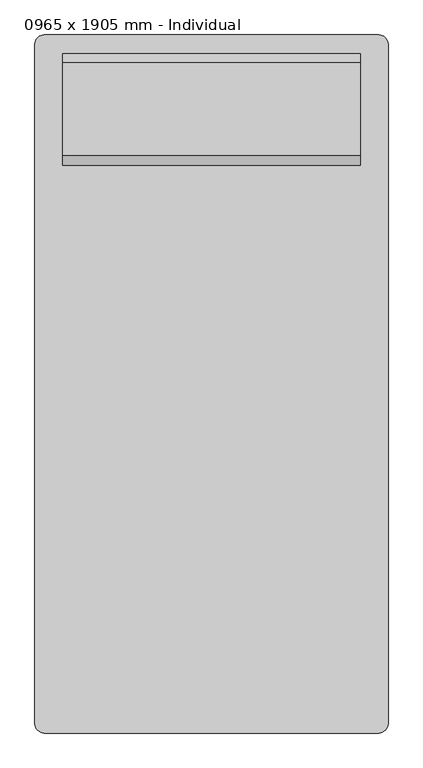
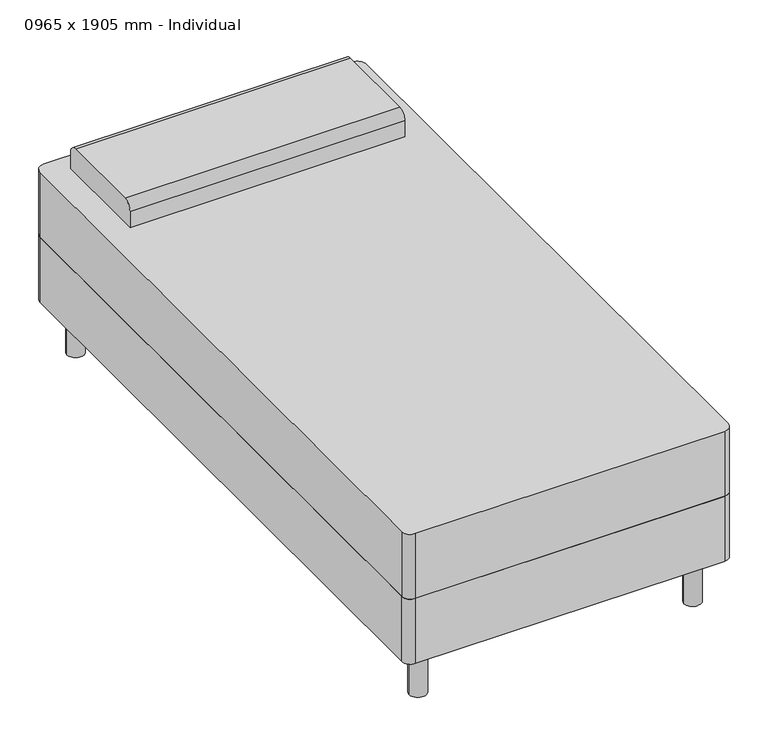
"""IFC4 building model written with IfcOpenShell, lengths in millimetres: furniture geometry, Cama-Estándar : 0965 x 1905 mm - Individual."""

import ifcopenshell
import ifcopenshell.guid

model = None  # the IFC model being written
_history = None  # IfcOwnerHistory: only IFC2X3 demands one
_inside = {}  # id of a spatial element -> (the spatial element, [elements in it])
_under = {}  # id of a project, library or spatial element -> (it, [spatial elements below it])
_declared = {}  # id of a project -> (the project, [libraries it declares])
_typed = {}  # id of a type object -> (the type object, [elements of that type])
_made_of = {}  # id of a material, layer set ... -> (it, [elements and type objects made of it])


def new_model(schema):
    """Start an empty IFC model of exactly this schema.

    Asked for "IFC4X3", IfcOpenShell would pick the latest addendum, in which some entities
    have other attributes; the version numbers below select the first issue.
    IFC2X3 requires an IfcOwnerHistory on every rooted entity: one is made here for all.
    """
    global model, _history
    if schema == "IFC4X3":
        model = ifcopenshell.file(schema_version=(4, 3, 0, 0))
    else:
        model = ifcopenshell.file(schema=schema)
    _inside.clear()
    _under.clear()
    _declared.clear()
    _typed.clear()
    _made_of.clear()
    _history = None
    if model.schema == "IFC2X3":
        org = make("IfcOrganization", Name="unknown")
        user = make(
            "IfcPersonAndOrganization",
            ThePerson=make("IfcPerson", FamilyName="unknown"),
            TheOrganization=org,
        )
        app = make(
            "IfcApplication",
            ApplicationDeveloper=org,
            Version="unknown",
            ApplicationFullName="unknown",
            ApplicationIdentifier="unknown",
        )
        _history = make(
            "IfcOwnerHistory",
            OwningUser=user,
            OwningApplication=app,
            ChangeAction="ADDED",
            CreationDate=0,
        )
    return model


def make(cls, **values):
    """One entity of the class cls with the attributes given. An attribute that is None is left unset."""
    return model.create_entity(
        cls, **{name: value for name, value in values.items() if value is not None}
    )


def rooted(cls, **values):
    """An entity with a GlobalId (a new one), such as an element, a storey or a relation."""
    return make(cls, GlobalId=ifcopenshell.guid.new(), OwnerHistory=_history, **values)


def si_unit(unit_type, name, prefix=None):
    """IfcSIUnit, for example si_unit("LENGTHUNIT", "METRE", prefix="MILLI")."""
    return make("IfcSIUnit", UnitType=unit_type, Prefix=prefix, Name=name)


def assignment(units):
    """IfcUnitAssignment: the units of a project."""
    return None if units is None else make("IfcUnitAssignment", Units=units)


def point(xyz):
    """IfcCartesianPoint."""
    return None if xyz is None else make("IfcCartesianPoint", Coordinates=xyz)


def direction(xyz):
    """IfcDirection."""
    return None if xyz is None else make("IfcDirection", DirectionRatios=xyz)


def frame(location, z_axis=None, x_axis=None):
    """IfcAxis2Placement3D, a coordinate frame: its origin and axes. An axis left out is left unset."""
    return make(
        "IfcAxis2Placement3D",
        Location=point(location),
        Axis=direction(z_axis),
        RefDirection=direction(x_axis),
    )


def frame_2d(location, x_axis=None):
    """IfcAxis2Placement2D, a coordinate frame in the plane: its origin and x axis."""
    return make(
        "IfcAxis2Placement2D", Location=point(location), RefDirection=direction(x_axis)
    )


def origin():
    """The frame at (0, 0, 0) with its axes left unset."""
    return frame((0.0, 0.0, 0.0))


def origin_with_axes():
    """The frame at (0, 0, 0) with the z axis (0, 0, 1) and the x axis (1, 0, 0) written out."""
    return frame((0.0, 0.0, 0.0), z_axis=(0.0, 0.0, 1.0), x_axis=(1.0, 0.0, 0.0))


def place(relative_to, where):
    """IfcLocalPlacement: puts the frame where relative to a parent placement (None: the world)."""
    return make(
        "IfcLocalPlacement", PlacementRelTo=relative_to, RelativePlacement=where
    )


def context(
    kind, dimensions, precision=None, world=None, true_north=None, identifier=None
):
    """IfcGeometricRepresentationContext, for example the 3D "Model" context."""
    return make(
        "IfcGeometricRepresentationContext",
        ContextIdentifier=identifier,
        ContextType=kind,
        CoordinateSpaceDimension=dimensions,
        Precision=precision,
        WorldCoordinateSystem=world,
        TrueNorth=true_north,
    )


def project(units=None, contexts=None):
    """IfcProject with its units and contexts."""
    return rooted(
        "IfcProject",
        Name="project",
        RepresentationContexts=contexts,
        UnitsInContext=assignment(units),
    )


def spatial(cls, under=None, at=None, **own):
    """A site, building, storey or space (cls), placed at a placement, below another one or the project."""
    s = rooted(cls, ObjectPlacement=at, **own)
    if under is not None:
        _under.setdefault(under.id(), (under, []))[1].append(s)
    return s


def polyline(points):
    """IfcPolyline through the points."""
    return make("IfcPolyline", Points=[point(p) for p in points])


def circle_curve(where, radius):
    """IfcCircle in the frame where."""
    return make("IfcCircle", Position=where, Radius=radius)


def trimmed(basis, trim1, trim2, sense, master):
    """IfcTrimmedCurve: the piece of a basis curve between two trims."""
    return make(
        "IfcTrimmedCurve",
        BasisCurve=basis,
        Trim1=trim1,
        Trim2=trim2,
        SenseAgreement=sense,
        MasterRepresentation=master,
    )


def segment(curve, same_sense, transition):
    """IfcCompositeCurveSegment."""
    return make(
        "IfcCompositeCurveSegment",
        Transition=transition,
        SameSense=same_sense,
        ParentCurve=curve,
    )


def composite_curve(segments, self_intersect=None):
    """IfcCompositeCurve: segments joined end to end."""
    return make("IfcCompositeCurve", Segments=segments, SelfIntersect=self_intersect)


def outline(outer, holes=None, kind="AREA"):
    """IfcArbitraryClosedProfileDef: a profile drawn as a closed curve; with holes, ...WithVoids."""
    if holes is None:
        return make("IfcArbitraryClosedProfileDef", ProfileType=kind, OuterCurve=outer)
    return make(
        "IfcArbitraryProfileDefWithVoids",
        ProfileType=kind,
        OuterCurve=outer,
        InnerCurves=holes,
    )


def extrude(swept, where, along, depth):
    """IfcExtrudedAreaSolid: the profile swept, set in the frame where, extruded along a direction by depth."""
    return make(
        "IfcExtrudedAreaSolid",
        SweptArea=swept,
        Position=where,
        ExtrudedDirection=direction(along),
        Depth=depth,
    )


def shape(context_of_items, identifier, shape_type, items):
    """IfcShapeRepresentation: the items that make up one representation, for example the "Body"."""
    return make(
        "IfcShapeRepresentation",
        ContextOfItems=context_of_items,
        RepresentationIdentifier=identifier,
        RepresentationType=shape_type,
        Items=items,
    )


def source(mapping_origin, context_of_items, identifier, shape_type, items):
    """IfcRepresentationMap: a shape defined once, which mapped items show again and again."""
    return make(
        "IfcRepresentationMap",
        MappingOrigin=mapping_origin,
        MappedRepresentation=shape(context_of_items, identifier, shape_type, items),
    )


def transform(
    local_origin,
    x_axis=None,
    y_axis=None,
    z_axis=None,
    scale=None,
    scale2=None,
    scale3=None,
    uniform=True,
):
    """IfcCartesianTransformationOperator3D, or its non-uniform kind. x_axis, y_axis, z_axis: its Axis1, 2, 3."""
    if uniform:
        return make(
            "IfcCartesianTransformationOperator3D",
            Axis1=direction(x_axis),
            Axis2=direction(y_axis),
            LocalOrigin=point(local_origin),
            Scale=scale,
            Axis3=direction(z_axis),
        )
    return make(
        "IfcCartesianTransformationOperator3DnonUniform",
        Axis1=direction(x_axis),
        Axis2=direction(y_axis),
        LocalOrigin=point(local_origin),
        Scale=scale,
        Axis3=direction(z_axis),
        Scale2=scale2,
        Scale3=scale3,
    )


def mapped(mapping_source, mapping_target):
    """IfcMappedItem: shows the shape of a source again, moved by a transform."""
    return make(
        "IfcMappedItem", MappingSource=mapping_source, MappingTarget=mapping_target
    )


def made_of(thing, what):
    """Note that an element or type object is made of a material, layer set ...; save() writes the relation."""
    if what is not None:
        _made_of.setdefault(what.id(), (what, []))[1].append(thing)
    return thing


def element(
    cls,
    number,
    at=None,
    inside=None,
    cuts=None,
    type_object=None,
    material=None,
    context=None,
    identifier="Body",
    shape_type=None,
    held_by="IfcProductDefinitionShape",
    body=None,
    shapes=None,
    **own,
):
    """One element of the class cls, such as IfcWall. Its Tag is "e" and its number.

    at: its placement. inside: the storey or other place that contains it. cuts: it is an
    opening in that element (IfcRelVoidsElement). A single representation is given by context,
    identifier, shape_type and body (its items); several are given by shapes. held_by: the class
    of the entity that holds the representations. save() writes the other relations.
    """
    e = rooted(cls, Tag="e%d" % number, ObjectPlacement=at, **own)
    if body is not None:
        shapes = [shape(context, identifier, shape_type, body)]
    if shapes is not None:
        e.Representation = make(held_by, Representations=shapes)
    if inside is not None:
        _inside.setdefault(inside.id(), (inside, []))[1].append(e)
    if cuts is not None:
        rooted(
            "IfcRelVoidsElement", RelatingBuildingElement=cuts, RelatedOpeningElement=e
        )
    if type_object is not None:
        _typed.setdefault(type_object.id(), (type_object, []))[1].append(e)
    return made_of(e, material)


def aggregate(whole, parts):
    """IfcRelAggregates: a whole, such as a stair, and the parts it consists of."""
    return rooted("IfcRelAggregates", RelatingObject=whole, RelatedObjects=parts)


def save(model, path):
    """Write the relations noted so far, then the file.

    IfcRelAggregates (storeys below a building ...), IfcRelContainedInSpatialStructure (elements
    in a storey), IfcRelDefinesByType, IfcRelAssociatesMaterial and IfcRelDeclares: one each for
    every whole, place, type object, material and project.
    """
    for whole, parts in _under.values():
        aggregate(whole, parts)
    for where, things in _inside.values():
        rooted(
            "IfcRelContainedInSpatialStructure",
            RelatedElements=things,
            RelatingStructure=where,
        )
    for kind, things in _typed.values():
        rooted("IfcRelDefinesByType", RelatedObjects=things, RelatingType=kind)
    for what, things in _made_of.values():
        rooted("IfcRelAssociatesMaterial", RelatedObjects=things, RelatingMaterial=what)
    for by, libraries in _declared.values():
        rooted("IfcRelDeclares", RelatingContext=by, RelatedDefinitions=libraries)
    model.write(path)


def furniture_0965_x_1905_mm_individual_fc46863d(model_context):
    return source(origin(), model_context, "Body", "SweptSolid", [
        extrude(outline(composite_curve([segment(polyline([(-211.0114754, -972.695082), (-211.0114754, 881.504918)]), True, "CONTINUOUS"), segment(trimmed(circle_curve(frame_2d((-185.6114754, 881.504918)), 25.4), [point((-211.0114754, 881.504918))], [point((-185.6114754, 906.904918))], False, "CARTESIAN"), True, "CONTINUOUS"), segment(polyline([(-185.6114754, 906.904918), (728.5885246, 906.904918)]), True, "CONTINUOUS"), segment(trimmed(circle_curve(frame_2d((728.5885246, 881.504918)), 25.4), [point((728.5885246, 906.904918))], [point((753.9885246, 881.504918))], False, "CARTESIAN"), True, "CONTINUOUS"), segment(polyline([(753.9885246, 881.504918), (753.9885246, -972.695082)]), True, "CONTINUOUS"), segment(trimmed(circle_curve(frame_2d((728.5885246, -972.695082)), 25.4), [point((753.9885246, -972.695082))], [point((728.5885246, -998.095082))], False, "CARTESIAN"), True, "CONTINUOUS"), segment(polyline([(728.5885246, -998.095082), (-185.6114754, -998.095082)]), True, "CONTINUOUS"), segment(trimmed(circle_curve(frame_2d((-185.6114754, -972.695082)), 25.4), [point((-185.6114754, -998.095082))], [point((-211.0114754, -972.695082))], False, "CARTESIAN"), True, "CONTINUOUS")], self_intersect=False)), frame((0.0, 0.0, 152.4), z_axis=(0.0, 0.0, 1.0), x_axis=(1.0, 0.0, 0.0)), (0.0, 0.0, 1.0), 203.2),
        extrude(outline(composite_curve([segment(polyline([(551.304918, 558.8), (551.304918, 609.6)]), True, "CONTINUOUS"), segment(trimmed(circle_curve(frame_2d((576.704918, 609.6)), 25.4), [point((551.304918, 609.6))], [point((576.704918, 635.0))], False, "CARTESIAN"), True, "CONTINUOUS"), segment(polyline([(576.704918, 635.0), (830.704918, 635.0)]), True, "CONTINUOUS"), segment(trimmed(circle_curve(frame_2d((830.704918, 609.6)), 25.4), [point((830.704918, 635.0))], [point((856.104918, 609.6))], False, "CARTESIAN"), True, "CONTINUOUS"), segment(polyline([(856.104918, 609.6), (856.104918, 558.8), (551.304918, 558.8)]), True, "CONTINUOUS")], self_intersect=False)), frame((-134.8114754, 0.0, 0.0), z_axis=(1.0, 0.0, 0.0), x_axis=(0.0, 1.0, 0.0)), (0.0, 0.0, 1.0), 812.6),
        extrude(outline(composite_curve([segment(trimmed(circle_curve(frame_2d((-134.8114754, 830.704918)), 25.4), [point((-160.2114754, 830.704918))], [point((-109.4114754, 830.704918))], False, "CARTESIAN"), True, "CONTINUOUS"), segment(trimmed(circle_curve(frame_2d((-134.8114754, 830.704918)), 25.4), [point((-109.4114754, 830.704918))], [point((-160.2114754, 830.704918))], False, "CARTESIAN"), True, "CONTINUOUS")], self_intersect=False)), origin_with_axes(), (0.0, 0.0, 1.0), 152.4),
        extrude(outline(composite_curve([segment(trimmed(circle_curve(frame_2d((677.7885246, 830.704918)), 25.4), [point((652.3885246, 830.704918))], [point((703.1885246, 830.704918))], False, "CARTESIAN"), True, "CONTINUOUS"), segment(trimmed(circle_curve(frame_2d((677.7885246, 830.704918)), 25.4), [point((703.1885246, 830.704918))], [point((652.3885246, 830.704918))], False, "CARTESIAN"), True, "CONTINUOUS")], self_intersect=False)), origin_with_axes(), (0.0, 0.0, 1.0), 152.4),
        extrude(outline(composite_curve([segment(trimmed(circle_curve(frame_2d((677.7885246, -921.895082)), 25.4), [point((652.3885246, -921.895082))], [point((703.1885246, -921.895082))], False, "CARTESIAN"), True, "CONTINUOUS"), segment(trimmed(circle_curve(frame_2d((677.7885246, -921.895082)), 25.4), [point((703.1885246, -921.895082))], [point((652.3885246, -921.895082))], False, "CARTESIAN"), True, "CONTINUOUS")], self_intersect=False)), origin_with_axes(), (0.0, 0.0, 1.0), 152.4),
        extrude(outline(composite_curve([segment(trimmed(circle_curve(frame_2d((-134.8114754, -921.895082)), 25.4), [point((-160.2114754, -921.895082))], [point((-109.4114754, -921.895082))], False, "CARTESIAN"), True, "CONTINUOUS"), segment(trimmed(circle_curve(frame_2d((-134.8114754, -921.895082)), 25.4), [point((-109.4114754, -921.895082))], [point((-160.2114754, -921.895082))], False, "CARTESIAN"), True, "CONTINUOUS")], self_intersect=False)), origin_with_axes(), (0.0, 0.0, 1.0), 152.4),
        extrude(outline(composite_curve([segment(polyline([(-185.6114754, 906.904918), (728.5885246, 906.904918)]), True, "CONTINUOUS"), segment(trimmed(circle_curve(frame_2d((728.5885246, 881.504918)), 25.4), [point((728.5885246, 906.904918))], [point((753.9885246, 881.504918))], False, "CARTESIAN"), True, "CONTINUOUS"), segment(polyline([(753.9885246, 881.504918), (753.9885246, -972.695082)]), True, "CONTINUOUS"), segment(trimmed(circle_curve(frame_2d((728.5885246, -972.695082)), 25.4), [point((753.9885246, -972.695082))], [point((728.5885246, -998.095082))], False, "CARTESIAN"), True, "CONTINUOUS"), segment(polyline([(728.5885246, -998.095082), (-185.6114754, -998.095082)]), True, "CONTINUOUS"), segment(trimmed(circle_curve(frame_2d((-185.6114754, -972.695082)), 25.4), [point((-185.6114754, -998.095082))], [point((-211.0114754, -972.695082))], False, "CARTESIAN"), True, "CONTINUOUS"), segment(polyline([(-211.0114754, -972.695082), (-211.0114754, 881.504918)]), True, "CONTINUOUS"), segment(trimmed(circle_curve(frame_2d((-185.6114754, 881.504918)), 25.4), [point((-211.0114754, 881.504918))], [point((-185.6114754, 906.904918))], False, "CARTESIAN"), True, "CONTINUOUS")], self_intersect=False)), frame((0.0, 0.0, 355.6), z_axis=(0.0, 0.0, 1.0), x_axis=(1.0, 0.0, 0.0)), (0.0, 0.0, 1.0), 203.2),
    ])


if __name__ == "__main__":
    model = new_model("IFC4")
    model_context = context("Model", 3, world=origin())
    ifc_project = project(units=[si_unit("LENGTHUNIT", "METRE", prefix="MILLI")], contexts=[model_context])
    site = spatial("IfcSite", under=ifc_project)
    building = spatial("IfcBuilding", under=site)
    placement = place(None, origin())
    furniture_0965_x_1905_mm_individual_shape = furniture_0965_x_1905_mm_individual_fc46863d(model_context)
    element("IfcFurniture", 1, ObjectType="Cama-Estándar : 0965 x 1905 mm - Individual", at=placement, inside=building, context=model_context, shape_type="MappedRepresentation", body=[
        mapped(furniture_0965_x_1905_mm_individual_shape, transform((0.0, 0.0, 0.0), x_axis=(1.0, 0.0, 0.0), y_axis=(0.0, 1.0, 0.0), z_axis=(0.0, 0.0, 1.0))),
    ])
    save(model, "model.ifc")

# Revit data of these elements
# Type "Cama-Estándar : 0965 x 1905 mm - Individual"
#   Longitud = 1.905 m
#   Anchura = 0.965 m
#   Máscara [instance default] = yes
#   Material de soporte = Metal - Cromo
#   Material de colchón = Textil - Blanco
#   Default Elevation = 0
# Element 1 (IfcFurniture, "Cama-Estándar : 0965 x 1905 mm - Individual")
#   Materials on its faces: "Metal - Cromo", "Textil - Blanco"
# Materials
#   "Metal - Cromo": class "Metal", colour RGB 17 17 17, transparency 0
#   "Textil - Blanco": class "Tela", colour RGB 247 247 239, transparency 0
